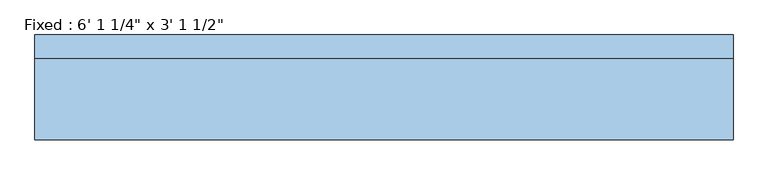
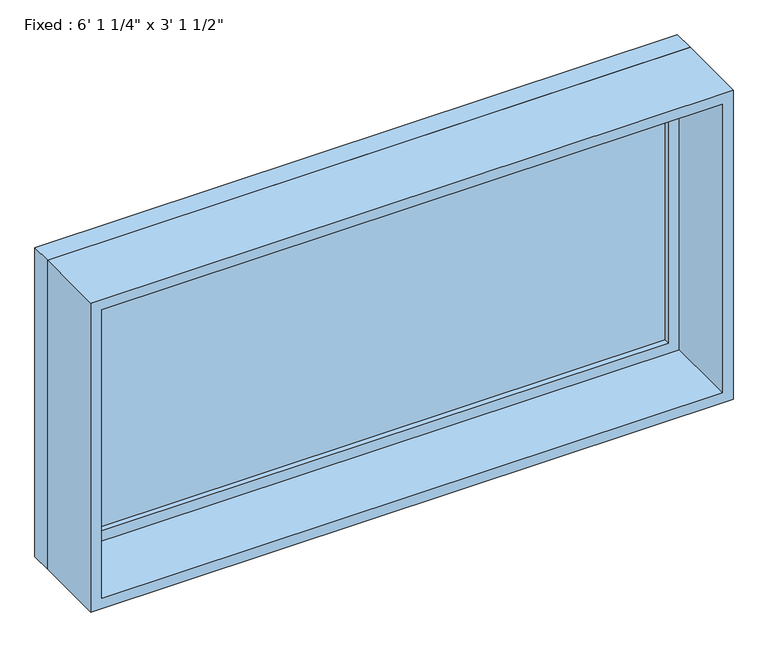
"""IFC4 building model written with IfcOpenShell, lengths in millimetres: window geometry."""

import ifcopenshell
import ifcopenshell.guid

model = None  # the IFC model being written
_history = None  # IfcOwnerHistory: only IFC2X3 demands one
_inside = {}  # id of a spatial element -> (the spatial element, [elements in it])
_under = {}  # id of a project, library or spatial element -> (it, [spatial elements below it])
_declared = {}  # id of a project -> (the project, [libraries it declares])
_typed = {}  # id of a type object -> (the type object, [elements of that type])
_made_of = {}  # id of a material, layer set ... -> (it, [elements and type objects made of it])


def new_model(schema):
    """Start an empty IFC model of exactly this schema.

    Asked for "IFC4X3", IfcOpenShell would pick the latest addendum, in which some entities
    have other attributes; the version numbers below select the first issue.
    IFC2X3 requires an IfcOwnerHistory on every rooted entity: one is made here for all.
    """
    global model, _history
    if schema == "IFC4X3":
        model = ifcopenshell.file(schema_version=(4, 3, 0, 0))
    else:
        model = ifcopenshell.file(schema=schema)
    _inside.clear()
    _under.clear()
    _declared.clear()
    _typed.clear()
    _made_of.clear()
    _history = None
    if model.schema == "IFC2X3":
        org = make("IfcOrganization", Name="unknown")
        user = make(
            "IfcPersonAndOrganization",
            ThePerson=make("IfcPerson", FamilyName="unknown"),
            TheOrganization=org,
        )
        app = make(
            "IfcApplication",
            ApplicationDeveloper=org,
            Version="unknown",
            ApplicationFullName="unknown",
            ApplicationIdentifier="unknown",
        )
        _history = make(
            "IfcOwnerHistory",
            OwningUser=user,
            OwningApplication=app,
            ChangeAction="ADDED",
            CreationDate=0,
        )
    return model


def make(cls, **values):
    """One entity of the class cls with the attributes given. An attribute that is None is left unset."""
    return model.create_entity(
        cls, **{name: value for name, value in values.items() if value is not None}
    )


def rooted(cls, **values):
    """An entity with a GlobalId (a new one), such as an element, a storey or a relation."""
    return make(cls, GlobalId=ifcopenshell.guid.new(), OwnerHistory=_history, **values)


def si_unit(unit_type, name, prefix=None):
    """IfcSIUnit, for example si_unit("LENGTHUNIT", "METRE", prefix="MILLI")."""
    return make("IfcSIUnit", UnitType=unit_type, Prefix=prefix, Name=name)


def assignment(units):
    """IfcUnitAssignment: the units of a project."""
    return None if units is None else make("IfcUnitAssignment", Units=units)


def point(xyz):
    """IfcCartesianPoint."""
    return None if xyz is None else make("IfcCartesianPoint", Coordinates=xyz)


def direction(xyz):
    """IfcDirection."""
    return None if xyz is None else make("IfcDirection", DirectionRatios=xyz)


def frame(location, z_axis=None, x_axis=None):
    """IfcAxis2Placement3D, a coordinate frame: its origin and axes. An axis left out is left unset."""
    return make(
        "IfcAxis2Placement3D",
        Location=point(location),
        Axis=direction(z_axis),
        RefDirection=direction(x_axis),
    )


def origin():
    """The frame at (0, 0, 0) with its axes left unset."""
    return frame((0.0, 0.0, 0.0))


def place(relative_to, where):
    """IfcLocalPlacement: puts the frame where relative to a parent placement (None: the world)."""
    return make(
        "IfcLocalPlacement", PlacementRelTo=relative_to, RelativePlacement=where
    )


def context(
    kind, dimensions, precision=None, world=None, true_north=None, identifier=None
):
    """IfcGeometricRepresentationContext, for example the 3D "Model" context."""
    return make(
        "IfcGeometricRepresentationContext",
        ContextIdentifier=identifier,
        ContextType=kind,
        CoordinateSpaceDimension=dimensions,
        Precision=precision,
        WorldCoordinateSystem=world,
        TrueNorth=true_north,
    )


def project(units=None, contexts=None):
    """IfcProject with its units and contexts."""
    return rooted(
        "IfcProject",
        Name="project",
        RepresentationContexts=contexts,
        UnitsInContext=assignment(units),
    )


def spatial(cls, under=None, at=None, **own):
    """A site, building, storey or space (cls), placed at a placement, below another one or the project."""
    s = rooted(cls, ObjectPlacement=at, **own)
    if under is not None:
        _under.setdefault(under.id(), (under, []))[1].append(s)
    return s


def polyline(points):
    """IfcPolyline through the points."""
    return make("IfcPolyline", Points=[point(p) for p in points])


def outline(outer, holes=None, kind="AREA"):
    """IfcArbitraryClosedProfileDef: a profile drawn as a closed curve; with holes, ...WithVoids."""
    if holes is None:
        return make("IfcArbitraryClosedProfileDef", ProfileType=kind, OuterCurve=outer)
    return make(
        "IfcArbitraryProfileDefWithVoids",
        ProfileType=kind,
        OuterCurve=outer,
        InnerCurves=holes,
    )


def extrude(swept, where, along, depth):
    """IfcExtrudedAreaSolid: the profile swept, set in the frame where, extruded along a direction by depth."""
    return make(
        "IfcExtrudedAreaSolid",
        SweptArea=swept,
        Position=where,
        ExtrudedDirection=direction(along),
        Depth=depth,
    )


def shape(context_of_items, identifier, shape_type, items):
    """IfcShapeRepresentation: the items that make up one representation, for example the "Body"."""
    return make(
        "IfcShapeRepresentation",
        ContextOfItems=context_of_items,
        RepresentationIdentifier=identifier,
        RepresentationType=shape_type,
        Items=items,
    )


def source(mapping_origin, context_of_items, identifier, shape_type, items):
    """IfcRepresentationMap: a shape defined once, which mapped items show again and again."""
    return make(
        "IfcRepresentationMap",
        MappingOrigin=mapping_origin,
        MappedRepresentation=shape(context_of_items, identifier, shape_type, items),
    )


def transform(
    local_origin,
    x_axis=None,
    y_axis=None,
    z_axis=None,
    scale=None,
    scale2=None,
    scale3=None,
    uniform=True,
):
    """IfcCartesianTransformationOperator3D, or its non-uniform kind. x_axis, y_axis, z_axis: its Axis1, 2, 3."""
    if uniform:
        return make(
            "IfcCartesianTransformationOperator3D",
            Axis1=direction(x_axis),
            Axis2=direction(y_axis),
            LocalOrigin=point(local_origin),
            Scale=scale,
            Axis3=direction(z_axis),
        )
    return make(
        "IfcCartesianTransformationOperator3DnonUniform",
        Axis1=direction(x_axis),
        Axis2=direction(y_axis),
        LocalOrigin=point(local_origin),
        Scale=scale,
        Axis3=direction(z_axis),
        Scale2=scale2,
        Scale3=scale3,
    )


def mapped(mapping_source, mapping_target):
    """IfcMappedItem: shows the shape of a source again, moved by a transform."""
    return make(
        "IfcMappedItem", MappingSource=mapping_source, MappingTarget=mapping_target
    )


def made_of(thing, what):
    """Note that an element or type object is made of a material, layer set ...; save() writes the relation."""
    if what is not None:
        _made_of.setdefault(what.id(), (what, []))[1].append(thing)
    return thing


def element(
    cls,
    number,
    at=None,
    inside=None,
    cuts=None,
    type_object=None,
    material=None,
    context=None,
    identifier="Body",
    shape_type=None,
    held_by="IfcProductDefinitionShape",
    body=None,
    shapes=None,
    **own,
):
    """One element of the class cls, such as IfcWall. Its Tag is "e" and its number.

    at: its placement. inside: the storey or other place that contains it. cuts: it is an
    opening in that element (IfcRelVoidsElement). A single representation is given by context,
    identifier, shape_type and body (its items); several are given by shapes. held_by: the class
    of the entity that holds the representations. save() writes the other relations.
    """
    e = rooted(cls, Tag="e%d" % number, ObjectPlacement=at, **own)
    if body is not None:
        shapes = [shape(context, identifier, shape_type, body)]
    if shapes is not None:
        e.Representation = make(held_by, Representations=shapes)
    if inside is not None:
        _inside.setdefault(inside.id(), (inside, []))[1].append(e)
    if cuts is not None:
        rooted(
            "IfcRelVoidsElement", RelatingBuildingElement=cuts, RelatedOpeningElement=e
        )
    if type_object is not None:
        _typed.setdefault(type_object.id(), (type_object, []))[1].append(e)
    return made_of(e, material)


def aggregate(whole, parts):
    """IfcRelAggregates: a whole, such as a stair, and the parts it consists of."""
    return rooted("IfcRelAggregates", RelatingObject=whole, RelatedObjects=parts)


def save(model, path):
    """Write the relations noted so far, then the file.

    IfcRelAggregates (storeys below a building ...), IfcRelContainedInSpatialStructure (elements
    in a storey), IfcRelDefinesByType, IfcRelAssociatesMaterial and IfcRelDeclares: one each for
    every whole, place, type object, material and project.
    """
    for whole, parts in _under.values():
        aggregate(whole, parts)
    for where, things in _inside.values():
        rooted(
            "IfcRelContainedInSpatialStructure",
            RelatedElements=things,
            RelatingStructure=where,
        )
    for kind, things in _typed.values():
        rooted("IfcRelDefinesByType", RelatedObjects=things, RelatingType=kind)
    for what, things in _made_of.values():
        rooted("IfcRelAssociatesMaterial", RelatedObjects=things, RelatingMaterial=what)
    for by, libraries in _declared.values():
        rooted("IfcRelDeclares", RelatingContext=by, RelatedDefinitions=libraries)
    model.write(path)


def window_d41c44e1(model_context):
    return source(origin(), model_context, "Body", "SweptSolid", [
        extrude(outline(polyline([(828.675, 92.075), (-904.875, 92.075), (-904.875, 104.775), (828.675, 104.775), (828.675, 92.075)])), frame((0.0, 0.0, 1257.3), z_axis=(0.0, 0.0, 1.0), x_axis=(1.0, 0.0, 0.0)), (0.0, 0.0, 1.0), 819.15),
        extrude(outline(polyline([(2120.9, -949.325), (1212.85, -949.325), (1212.85, 873.125), (2120.9, 873.125), (2120.9, -949.325)]), holes=[polyline([(2076.45, -904.875), (2076.45, 828.675), (1257.3, 828.675), (1257.3, -904.875), (2076.45, -904.875)])]), frame((0.0, 76.2, 0.0), z_axis=(0.0, 1.0, 0.0), x_axis=(0.0, 0.0, 1.0)), (0.0, 0.0, 1.0), 44.45),
        extrude(outline(polyline([(2139.95, -968.375), (1193.8, -968.375), (1193.8, 892.175), (2139.95, 892.175), (2139.95, -968.375)]), holes=[polyline([(2108.2, -936.625), (2108.2, 860.425), (1225.55, 860.425), (1225.55, -936.625), (2108.2, -936.625)])]), frame((0.0, -139.7, 0.0), z_axis=(0.0, 1.0, 0.0), x_axis=(0.0, 0.0, 1.0)), (0.0, 0.0, 1.0), 215.9),
        extrude(outline(polyline([(2139.95, 892.175), (2139.95, -968.375), (1193.8, -968.375), (1193.8, 892.175), (2139.95, 892.175)]), holes=[polyline([(2120.9, 873.125), (1212.85, 873.125), (1212.85, -949.325), (2120.9, -949.325), (2120.9, 873.125)])]), frame((0.0, 76.2, 0.0), z_axis=(0.0, 1.0, 0.0), x_axis=(0.0, 0.0, 1.0)), (0.0, 0.0, 1.0), 63.5),
    ])


if __name__ == "__main__":
    model = new_model("IFC4")
    model_context = context("Model", 3, world=origin())
    ifc_project = project(units=[si_unit("LENGTHUNIT", "METRE", prefix="MILLI")], contexts=[model_context])
    site = spatial("IfcSite", under=ifc_project)
    building = spatial("IfcBuilding", under=site)
    placement = place(None, origin())
    window_shape = window_d41c44e1(model_context)
    element("IfcWindow", 1, ObjectType="Fixed : 6' 1 1/4\" x 3' 1 1/2\"", at=placement, inside=building, context=model_context, shape_type="MappedRepresentation", body=[
        mapped(window_shape, transform((0.0, 0.0, 0.0), x_axis=(1.0, 0.0, 0.0), y_axis=(0.0, 1.0, 0.0), z_axis=(0.0, 0.0, 1.0))),
    ])
    save(model, "model.ifc")

# Revit data of these elements
# Type "Fixed : 6' 1 1/4\" x 3' 1 1/2\""
#   Type Mark = "21"
#   Assembly Code = "B2020100"
#   Height = 3' - 1 1/4"
#   Default Sill Height = 3' - 11"
#   Width = 6' - 1 1/4"
#   Window Inset = 0' - 0 3/4"
#   Glass Pane Material = Glass
#   Sash Material = accent 2
#   Wall Closure = (empty or 0)
# Element 1 (IfcWindow, "Fixed : 6' 1 1/4\" x 3' 1 1/2\"")
#   Materials on its faces: "accent 2", "Glass"
# Materials
#   "Glass": class "Glass", colour RGB 236 240 239, transparency 0.85, Description = "Soda Lime Glass", Cost = 0
#   "accent 2": class "Wood", colour RGB 80 80 80, transparency 0, Description = "Wood framing, thermal airspace", Cost = 0
